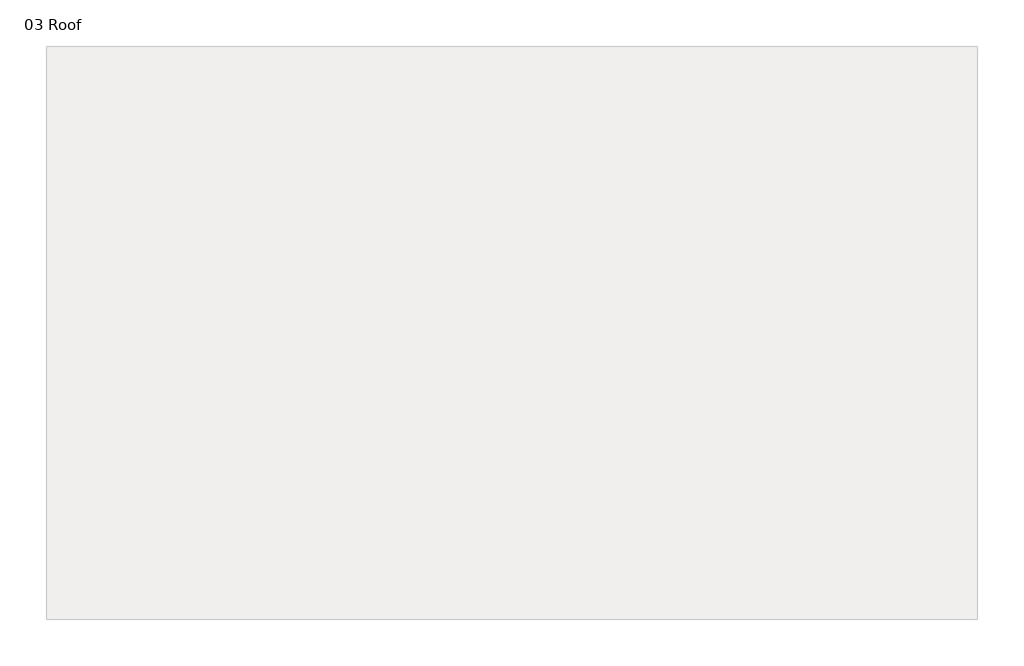
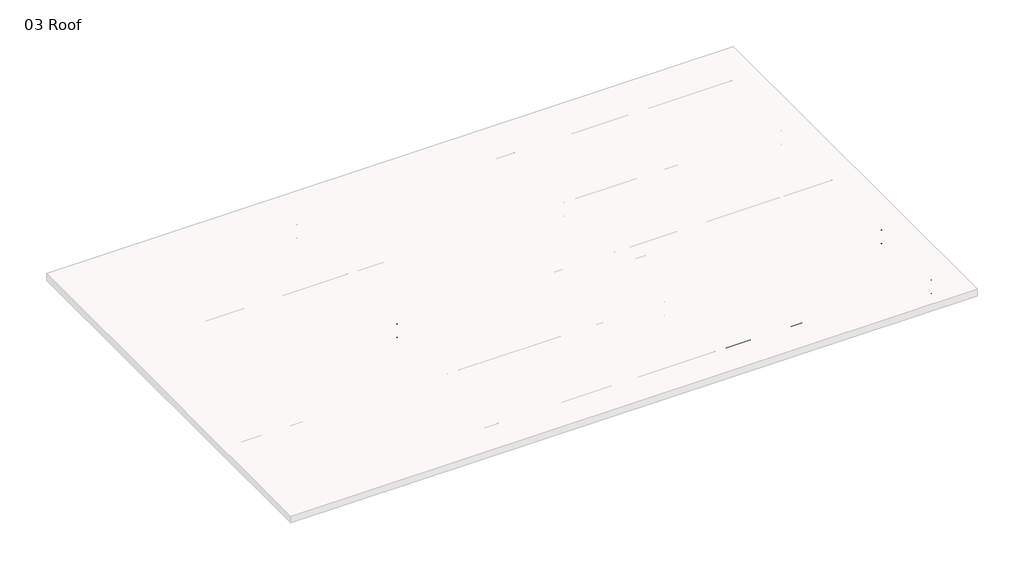
# One storey, part 2 of 4: 101 beams.
"""IFC4 building model written with IfcOpenShell, lengths in millimetres."""

import ifcopenshell
import ifcopenshell.guid

model = None  # the IFC model being written
_history = None  # IfcOwnerHistory: only IFC2X3 demands one
_inside = {}  # id of a spatial element -> (the spatial element, [elements in it])
_under = {}  # id of a project, library or spatial element -> (it, [spatial elements below it])
_declared = {}  # id of a project -> (the project, [libraries it declares])
_typed = {}  # id of a type object -> (the type object, [elements of that type])
_made_of = {}  # id of a material, layer set ... -> (it, [elements and type objects made of it])


def new_model(schema):
    """Start an empty IFC model of exactly this schema.

    Asked for "IFC4X3", IfcOpenShell would pick the latest addendum, in which some entities
    have other attributes; the version numbers below select the first issue.
    IFC2X3 requires an IfcOwnerHistory on every rooted entity: one is made here for all.
    """
    global model, _history
    if schema == "IFC4X3":
        model = ifcopenshell.file(schema_version=(4, 3, 0, 0))
    else:
        model = ifcopenshell.file(schema=schema)
    _inside.clear()
    _under.clear()
    _declared.clear()
    _typed.clear()
    _made_of.clear()
    _history = None
    if model.schema == "IFC2X3":
        org = make("IfcOrganization", Name="unknown")
        user = make(
            "IfcPersonAndOrganization",
            ThePerson=make("IfcPerson", FamilyName="unknown"),
            TheOrganization=org,
        )
        app = make(
            "IfcApplication",
            ApplicationDeveloper=org,
            Version="unknown",
            ApplicationFullName="unknown",
            ApplicationIdentifier="unknown",
        )
        _history = make(
            "IfcOwnerHistory",
            OwningUser=user,
            OwningApplication=app,
            ChangeAction="ADDED",
            CreationDate=0,
        )
    return model


def make(cls, **values):
    """One entity of the class cls with the attributes given. An attribute that is None is left unset."""
    return model.create_entity(
        cls, **{name: value for name, value in values.items() if value is not None}
    )


def rooted(cls, **values):
    """An entity with a GlobalId (a new one), such as an element, a storey or a relation."""
    return make(cls, GlobalId=ifcopenshell.guid.new(), OwnerHistory=_history, **values)


def si_unit(unit_type, name, prefix=None):
    """IfcSIUnit, for example si_unit("LENGTHUNIT", "METRE", prefix="MILLI")."""
    return make("IfcSIUnit", UnitType=unit_type, Prefix=prefix, Name=name)


def assignment(units):
    """IfcUnitAssignment: the units of a project."""
    return None if units is None else make("IfcUnitAssignment", Units=units)


def point(xyz):
    """IfcCartesianPoint."""
    return None if xyz is None else make("IfcCartesianPoint", Coordinates=xyz)


def direction(xyz):
    """IfcDirection."""
    return None if xyz is None else make("IfcDirection", DirectionRatios=xyz)


def frame(location, z_axis=None, x_axis=None):
    """IfcAxis2Placement3D, a coordinate frame: its origin and axes. An axis left out is left unset."""
    return make(
        "IfcAxis2Placement3D",
        Location=point(location),
        Axis=direction(z_axis),
        RefDirection=direction(x_axis),
    )


def frame_2d(location, x_axis=None):
    """IfcAxis2Placement2D, a coordinate frame in the plane: its origin and x axis."""
    return make(
        "IfcAxis2Placement2D", Location=point(location), RefDirection=direction(x_axis)
    )


def origin():
    """The frame at (0, 0, 0) with its axes left unset."""
    return frame((0.0, 0.0, 0.0))


def place(relative_to, where):
    """IfcLocalPlacement: puts the frame where relative to a parent placement (None: the world)."""
    return make(
        "IfcLocalPlacement", PlacementRelTo=relative_to, RelativePlacement=where
    )


def context(
    kind, dimensions, precision=None, world=None, true_north=None, identifier=None
):
    """IfcGeometricRepresentationContext, for example the 3D "Model" context."""
    return make(
        "IfcGeometricRepresentationContext",
        ContextIdentifier=identifier,
        ContextType=kind,
        CoordinateSpaceDimension=dimensions,
        Precision=precision,
        WorldCoordinateSystem=world,
        TrueNorth=true_north,
    )


def project(units=None, contexts=None):
    """IfcProject with its units and contexts."""
    return rooted(
        "IfcProject",
        Name="project",
        RepresentationContexts=contexts,
        UnitsInContext=assignment(units),
    )


def spatial(cls, under=None, at=None, **own):
    """A site, building, storey or space (cls), placed at a placement, below another one or the project."""
    s = rooted(cls, ObjectPlacement=at, **own)
    if under is not None:
        _under.setdefault(under.id(), (under, []))[1].append(s)
    return s


def polyline(points):
    """IfcPolyline through the points."""
    return make("IfcPolyline", Points=[point(p) for p in points])


def circle_curve(where, radius):
    """IfcCircle in the frame where."""
    return make("IfcCircle", Position=where, Radius=radius)


def trimmed(basis, trim1, trim2, sense, master):
    """IfcTrimmedCurve: the piece of a basis curve between two trims."""
    return make(
        "IfcTrimmedCurve",
        BasisCurve=basis,
        Trim1=trim1,
        Trim2=trim2,
        SenseAgreement=sense,
        MasterRepresentation=master,
    )


def segment(curve, same_sense, transition):
    """IfcCompositeCurveSegment."""
    return make(
        "IfcCompositeCurveSegment",
        Transition=transition,
        SameSense=same_sense,
        ParentCurve=curve,
    )


def composite_curve(segments, self_intersect=None):
    """IfcCompositeCurve: segments joined end to end."""
    return make("IfcCompositeCurve", Segments=segments, SelfIntersect=self_intersect)


def outline(outer, holes=None, kind="AREA"):
    """IfcArbitraryClosedProfileDef: a profile drawn as a closed curve; with holes, ...WithVoids."""
    if holes is None:
        return make("IfcArbitraryClosedProfileDef", ProfileType=kind, OuterCurve=outer)
    return make(
        "IfcArbitraryProfileDefWithVoids",
        ProfileType=kind,
        OuterCurve=outer,
        InnerCurves=holes,
    )


def extrude(swept, where, along, depth):
    """IfcExtrudedAreaSolid: the profile swept, set in the frame where, extruded along a direction by depth."""
    return make(
        "IfcExtrudedAreaSolid",
        SweptArea=swept,
        Position=where,
        ExtrudedDirection=direction(along),
        Depth=depth,
    )


def shape(context_of_items, identifier, shape_type, items):
    """IfcShapeRepresentation: the items that make up one representation, for example the "Body"."""
    return make(
        "IfcShapeRepresentation",
        ContextOfItems=context_of_items,
        RepresentationIdentifier=identifier,
        RepresentationType=shape_type,
        Items=items,
    )


def source(mapping_origin, context_of_items, identifier, shape_type, items):
    """IfcRepresentationMap: a shape defined once, which mapped items show again and again."""
    return make(
        "IfcRepresentationMap",
        MappingOrigin=mapping_origin,
        MappedRepresentation=shape(context_of_items, identifier, shape_type, items),
    )


def transform(
    local_origin,
    x_axis=None,
    y_axis=None,
    z_axis=None,
    scale=None,
    scale2=None,
    scale3=None,
    uniform=True,
):
    """IfcCartesianTransformationOperator3D, or its non-uniform kind. x_axis, y_axis, z_axis: its Axis1, 2, 3."""
    if uniform:
        return make(
            "IfcCartesianTransformationOperator3D",
            Axis1=direction(x_axis),
            Axis2=direction(y_axis),
            LocalOrigin=point(local_origin),
            Scale=scale,
            Axis3=direction(z_axis),
        )
    return make(
        "IfcCartesianTransformationOperator3DnonUniform",
        Axis1=direction(x_axis),
        Axis2=direction(y_axis),
        LocalOrigin=point(local_origin),
        Scale=scale,
        Axis3=direction(z_axis),
        Scale2=scale2,
        Scale3=scale3,
    )


def mapped(mapping_source, mapping_target):
    """IfcMappedItem: shows the shape of a source again, moved by a transform."""
    return make(
        "IfcMappedItem", MappingSource=mapping_source, MappingTarget=mapping_target
    )


def made_of(thing, what):
    """Note that an element or type object is made of a material, layer set ...; save() writes the relation."""
    if what is not None:
        _made_of.setdefault(what.id(), (what, []))[1].append(thing)
    return thing


def element(
    cls,
    number,
    at=None,
    inside=None,
    cuts=None,
    type_object=None,
    material=None,
    context=None,
    identifier="Body",
    shape_type=None,
    held_by="IfcProductDefinitionShape",
    body=None,
    shapes=None,
    **own,
):
    """One element of the class cls, such as IfcWall. Its Tag is "e" and its number.

    at: its placement. inside: the storey or other place that contains it. cuts: it is an
    opening in that element (IfcRelVoidsElement). A single representation is given by context,
    identifier, shape_type and body (its items); several are given by shapes. held_by: the class
    of the entity that holds the representations. save() writes the other relations.
    """
    e = rooted(cls, Tag="e%d" % number, ObjectPlacement=at, **own)
    if body is not None:
        shapes = [shape(context, identifier, shape_type, body)]
    if shapes is not None:
        e.Representation = make(held_by, Representations=shapes)
    if inside is not None:
        _inside.setdefault(inside.id(), (inside, []))[1].append(e)
    if cuts is not None:
        rooted(
            "IfcRelVoidsElement", RelatingBuildingElement=cuts, RelatedOpeningElement=e
        )
    if type_object is not None:
        _typed.setdefault(type_object.id(), (type_object, []))[1].append(e)
    return made_of(e, material)


def aggregate(whole, parts):
    """IfcRelAggregates: a whole, such as a stair, and the parts it consists of."""
    return rooted("IfcRelAggregates", RelatingObject=whole, RelatedObjects=parts)


def save(model, path):
    """Write the relations noted so far, then the file.

    IfcRelAggregates (storeys below a building ...), IfcRelContainedInSpatialStructure (elements
    in a storey), IfcRelDefinesByType, IfcRelAssociatesMaterial and IfcRelDeclares: one each for
    every whole, place, type object, material and project.
    """
    for whole, parts in _under.values():
        aggregate(whole, parts)
    for where, things in _inside.values():
        rooted(
            "IfcRelContainedInSpatialStructure",
            RelatedElements=things,
            RelatingStructure=where,
        )
    for kind, things in _typed.values():
        rooted("IfcRelDefinesByType", RelatedObjects=things, RelatingType=kind)
    for what, things in _made_of.values():
        rooted("IfcRelAssociatesMaterial", RelatedObjects=things, RelatingMaterial=what)
    for by, libraries in _declared.values():
        rooted("IfcRelDeclares", RelatingContext=by, RelatedDefinitions=libraries)
    model.write(path)


def ub_universal_beam_305x165x40ub_24de31be(model_context):
    return source(origin(), model_context, "Body", "SweptSolid", [
        extrude(outline(composite_curve([segment(polyline([(82.5, -141.5), (82.5, -151.7), (-82.5, -151.7), (-82.5, -141.5), (-11.9, -141.5)]), True, "CONTINUOUS"), segment(trimmed(circle_curve(frame_2d((-11.9, -132.6)), 8.9), [point((-11.9, -141.5))], [point((-3.0, -132.6))], True, "CARTESIAN"), True, "CONTINUOUS"), segment(polyline([(-3.0, -132.6), (-3.0, 132.6)]), True, "CONTINUOUS"), segment(trimmed(circle_curve(frame_2d((-11.9, 132.6)), 8.9), [point((-3.0, 132.6))], [point((-11.9, 141.5))], True, "CARTESIAN"), True, "CONTINUOUS"), segment(polyline([(-11.9, 141.5), (-82.5, 141.5), (-82.5, 151.7), (82.5, 151.7), (82.5, 141.5), (11.9, 141.5)]), True, "CONTINUOUS"), segment(trimmed(circle_curve(frame_2d((11.9, 132.6)), 8.9), [point((11.9, 141.5))], [point((3.0, 132.6))], True, "CARTESIAN"), True, "CONTINUOUS"), segment(polyline([(3.0, 132.6), (3.0, -132.6)]), True, "CONTINUOUS"), segment(trimmed(circle_curve(frame_2d((11.9, -132.6)), 8.9), [point((3.0, -132.6))], [point((11.9, -141.5))], True, "CARTESIAN"), True, "CONTINUOUS"), segment(polyline([(11.9, -141.5), (82.5, -141.5)]), True, "CONTINUOUS")], self_intersect=False)), frame((-335.6, 0.0, 0.0), z_axis=(1.0, 0.0, 0.0), x_axis=(0.0, 1.0, 0.0)), (0.0, 0.0, 1.0), 671.2),
    ])


def ub_universal_beam_305x165x40ub_f67fc52f(model_context):
    return source(origin(), model_context, "Body", "SweptSolid", [
        extrude(outline(composite_curve([segment(polyline([(82.5, -141.5), (82.5, -151.7), (-82.5, -151.7), (-82.5, -141.5), (-11.9, -141.5)]), True, "CONTINUOUS"), segment(trimmed(circle_curve(frame_2d((-11.9, -132.6)), 8.9), [point((-11.9, -141.5))], [point((-3.0, -132.6))], True, "CARTESIAN"), True, "CONTINUOUS"), segment(polyline([(-3.0, -132.6), (-3.0, 132.6)]), True, "CONTINUOUS"), segment(trimmed(circle_curve(frame_2d((-11.9, 132.6)), 8.9), [point((-3.0, 132.6))], [point((-11.9, 141.5))], True, "CARTESIAN"), True, "CONTINUOUS"), segment(polyline([(-11.9, 141.5), (-82.5, 141.5), (-82.5, 151.7), (82.5, 151.7), (82.5, 141.5), (11.9, 141.5)]), True, "CONTINUOUS"), segment(trimmed(circle_curve(frame_2d((11.9, 132.6)), 8.9), [point((11.9, 141.5))], [point((3.0, 132.6))], True, "CARTESIAN"), True, "CONTINUOUS"), segment(polyline([(3.0, 132.6), (3.0, -132.6)]), True, "CONTINUOUS"), segment(trimmed(circle_curve(frame_2d((11.9, -132.6)), 8.9), [point((3.0, -132.6))], [point((11.9, -141.5))], True, "CARTESIAN"), True, "CONTINUOUS"), segment(polyline([(11.9, -141.5), (82.5, -141.5)]), True, "CONTINUOUS")], self_intersect=False)), frame((-7125.0, 0.0, 0.0), z_axis=(1.0, 0.0, 0.0), x_axis=(0.0, 1.0, 0.0)), (0.0, 0.0, 1.0), 14250.0),
    ])


def ub_universal_beam_305x165x40ub_26fb8d3a(model_context):
    return source(origin(), model_context, "Body", "SweptSolid", [
        extrude(outline(composite_curve([segment(polyline([(82.5, -141.5), (82.5, -151.7), (-82.5, -151.7), (-82.5, -141.5), (-11.9, -141.5)]), True, "CONTINUOUS"), segment(trimmed(circle_curve(frame_2d((-11.9, -132.6)), 8.9), [point((-11.9, -141.5))], [point((-3.0, -132.6))], True, "CARTESIAN"), True, "CONTINUOUS"), segment(polyline([(-3.0, -132.6), (-3.0, 132.6)]), True, "CONTINUOUS"), segment(trimmed(circle_curve(frame_2d((-11.9, 132.6)), 8.9), [point((-3.0, 132.6))], [point((-11.9, 141.5))], True, "CARTESIAN"), True, "CONTINUOUS"), segment(polyline([(-11.9, 141.5), (-82.5, 141.5), (-82.5, 151.7), (82.5, 151.7), (82.5, 141.5), (11.9, 141.5)]), True, "CONTINUOUS"), segment(trimmed(circle_curve(frame_2d((11.9, 132.6)), 8.9), [point((11.9, 141.5))], [point((3.0, 132.6))], True, "CARTESIAN"), True, "CONTINUOUS"), segment(polyline([(3.0, 132.6), (3.0, -132.6)]), True, "CONTINUOUS"), segment(trimmed(circle_curve(frame_2d((11.9, -132.6)), 8.9), [point((3.0, -132.6))], [point((11.9, -141.5))], True, "CARTESIAN"), True, "CONTINUOUS"), segment(polyline([(11.9, -141.5), (82.5, -141.5)]), True, "CONTINUOUS")], self_intersect=False)), frame((-347.8807825, 0.0, 0.0), z_axis=(1.0, 0.0, 0.0), x_axis=(0.0, 1.0, 0.0)), (0.0, 0.0, 1.0), 695.761565),
    ])


model = new_model("IFC4")

# Units and contexts
model_context = context("Model", 3, world=origin())
ifc_project = project(units=[si_unit("LENGTHUNIT", "METRE", prefix="MILLI")], contexts=[model_context])

# Site, building, storey
site = spatial("IfcSite", under=ifc_project)
building = spatial("IfcBuilding", under=site)
storey = spatial("IfcBuildingStorey", under=building, Name="03 Roof", Elevation=8000.0)

# Beams
placement = place(None, origin())
ub_universal_beam_305x165x40ub_shape = ub_universal_beam_305x165x40ub_24de31be(model_context)
element("IfcBeam", 1, ObjectType="UB-Universal Beam : 305x165x40UB", at=placement, inside=storey, context=model_context, shape_type="MappedRepresentation", body=[
    mapped(ub_universal_beam_305x165x40ub_shape, transform((-21151.5506826, 12261.9474871, 7500.0), x_axis=(0.0, 0.0, 1.0), y_axis=(0.0, -1.0, 0.0), z_axis=(1.0, 0.0, 0.0))),
])
element("IfcBeam", 2, ObjectType="UB-Universal Beam : 305x165x40UB", at=placement, inside=storey, context=model_context, shape_type="MappedRepresentation", body=[
    mapped(ub_universal_beam_305x165x40ub_shape, transform((-19964.0506826, 12261.9474871, 7500.0), x_axis=(0.0, 0.0, 1.0), y_axis=(0.0, -1.0, 0.0), z_axis=(1.0, 0.0, 0.0))),
])
element("IfcBeam", 3, ObjectType="UB-Universal Beam : 305x165x40UB", at=placement, inside=storey, context=model_context, shape_type="MappedRepresentation", body=[
    mapped(ub_universal_beam_305x165x40ub_shape, transform((-18776.5506826, 12261.9474871, 7500.0), x_axis=(0.0, 0.0, 1.0), y_axis=(0.0, -1.0, 0.0), z_axis=(1.0, 0.0, 0.0))),
])
element("IfcBeam", 4, ObjectType="UB-Universal Beam : 305x165x40UB", at=placement, inside=storey, context=model_context, shape_type="MappedRepresentation", body=[
    mapped(ub_universal_beam_305x165x40ub_shape, transform((-17589.0506826, 12261.9474871, 7500.0), x_axis=(0.0, 0.0, 1.0), y_axis=(0.0, -1.0, 0.0), z_axis=(1.0, 0.0, 0.0))),
])
element("IfcBeam", 5, ObjectType="UB-Universal Beam : 305x165x40UB", at=placement, inside=storey, context=model_context, shape_type="MappedRepresentation", body=[
    mapped(ub_universal_beam_305x165x40ub_shape, transform((-22339.0506826, 12261.9474871, 7500.0), x_axis=(0.0, 0.0, 1.0), y_axis=(0.0, -1.0, 0.0), z_axis=(1.0, 0.0, 0.0))),
])
element("IfcBeam", 6, ObjectType="UB-Universal Beam : 305x165x40UB", at=placement, inside=storey, context=model_context, shape_type="MappedRepresentation", body=[
    mapped(ub_universal_beam_305x165x40ub_shape, transform((-16401.5506826, 12261.9474871, 7500.0), x_axis=(0.0, 0.0, 1.0), y_axis=(0.0, -1.0, 0.0), z_axis=(1.0, 0.0, 0.0))),
])
element("IfcBeam", 7, ObjectType="UB-Universal Beam : 305x165x40UB", at=placement, inside=storey, context=model_context, shape_type="MappedRepresentation", body=[
    mapped(ub_universal_beam_305x165x40ub_shape, transform((-21151.5506826, 6271.8474871, 7500.0), x_axis=(0.0, 0.0, 1.0), y_axis=(0.0, -1.0, 0.0), z_axis=(1.0, 0.0, 0.0))),
])
element("IfcBeam", 8, ObjectType="UB-Universal Beam : 305x165x40UB", at=placement, inside=storey, context=model_context, shape_type="MappedRepresentation", body=[
    mapped(ub_universal_beam_305x165x40ub_shape, transform((-19964.0506826, 6271.8474871, 7500.0), x_axis=(0.0, 0.0, 1.0), y_axis=(0.0, -1.0, 0.0), z_axis=(1.0, 0.0, 0.0))),
])
element("IfcBeam", 9, ObjectType="UB-Universal Beam : 305x165x40UB", at=placement, inside=storey, context=model_context, shape_type="MappedRepresentation", body=[
    mapped(ub_universal_beam_305x165x40ub_shape, transform((-18776.5506826, 6271.8474871, 7500.0), x_axis=(0.0, 0.0, 1.0), y_axis=(0.0, -1.0, 0.0), z_axis=(1.0, 0.0, 0.0))),
])
element("IfcBeam", 10, ObjectType="UB-Universal Beam : 305x165x40UB", at=placement, inside=storey, context=model_context, shape_type="MappedRepresentation", body=[
    mapped(ub_universal_beam_305x165x40ub_shape, transform((-17589.0506826, 6271.8474871, 7500.0), x_axis=(0.0, 0.0, 1.0), y_axis=(0.0, -1.0, 0.0), z_axis=(1.0, 0.0, 0.0))),
])
element("IfcBeam", 11, ObjectType="UB-Universal Beam : 305x165x40UB", at=placement, inside=storey, context=model_context, shape_type="MappedRepresentation", body=[
    mapped(ub_universal_beam_305x165x40ub_shape, transform((-22339.0506826, 6271.8474871, 7500.0), x_axis=(0.0, 0.0, 1.0), y_axis=(0.0, -1.0, 0.0), z_axis=(1.0, 0.0, 0.0))),
])
element("IfcBeam", 12, ObjectType="UB-Universal Beam : 305x165x40UB", at=placement, inside=storey, context=model_context, shape_type="MappedRepresentation", body=[
    mapped(ub_universal_beam_305x165x40ub_shape, transform((-16401.5506826, 6271.8474871, 7500.0), x_axis=(0.0, 0.0, 1.0), y_axis=(0.0, -1.0, 0.0), z_axis=(1.0, 0.0, 0.0))),
])
element("IfcBeam", 13, ObjectType="UB-Universal Beam : 305x165x40UB", at=placement, inside=storey, context=model_context, shape_type="MappedRepresentation", body=[
    mapped(ub_universal_beam_305x165x40ub_shape, transform((20723.4493174, -5728.1525129, 7500.0), x_axis=(0.0, 0.0, 1.0), y_axis=(0.0, -1.0, 0.0), z_axis=(1.0, 0.0, 0.0))),
])
element("IfcBeam", 14, ObjectType="UB-Universal Beam : 305x165x40UB", at=placement, inside=storey, context=model_context, shape_type="MappedRepresentation", body=[
    mapped(ub_universal_beam_305x165x40ub_shape, transform((8848.4493174, -5728.1525129, 7500.0), x_axis=(0.0, 0.0, 1.0), y_axis=(0.0, -1.0, 0.0), z_axis=(1.0, 0.0, 0.0))),
])
element("IfcBeam", 15, ObjectType="UB-Universal Beam : 305x165x40UB", at=placement, inside=storey, context=model_context, shape_type="MappedRepresentation", body=[
    mapped(ub_universal_beam_305x165x40ub_shape, transform((19535.9493174, -5728.1525129, 7500.0), x_axis=(0.0, 0.0, 1.0), y_axis=(0.0, -1.0, 0.0), z_axis=(1.0, 0.0, 0.0))),
])
element("IfcBeam", 16, ObjectType="UB-Universal Beam : 305x165x40UB", at=placement, inside=storey, context=model_context, shape_type="MappedRepresentation", body=[
    mapped(ub_universal_beam_305x165x40ub_shape, transform((10035.9493174, -5728.1525129, 7500.0), x_axis=(0.0, 0.0, 1.0), y_axis=(0.0, -1.0, 0.0), z_axis=(1.0, 0.0, 0.0))),
])
element("IfcBeam", 17, ObjectType="UB-Universal Beam : 305x165x40UB", at=placement, inside=storey, context=model_context, shape_type="MappedRepresentation", body=[
    mapped(ub_universal_beam_305x165x40ub_shape, transform((18348.4493174, -5728.1525129, 7500.0), x_axis=(0.0, 0.0, 1.0), y_axis=(0.0, -1.0, 0.0), z_axis=(1.0, 0.0, 0.0))),
])
element("IfcBeam", 18, ObjectType="UB-Universal Beam : 305x165x40UB", at=placement, inside=storey, context=model_context, shape_type="MappedRepresentation", body=[
    mapped(ub_universal_beam_305x165x40ub_shape, transform((17160.9493174, -5728.1525129, 7500.0), x_axis=(0.0, 0.0, 1.0), y_axis=(0.0, -1.0, 0.0), z_axis=(1.0, 0.0, 0.0))),
])
element("IfcBeam", 19, ObjectType="UB-Universal Beam : 305x165x40UB", at=placement, inside=storey, context=model_context, shape_type="MappedRepresentation", body=[
    mapped(ub_universal_beam_305x165x40ub_shape, transform((21910.9493174, -5728.1525129, 7500.0), x_axis=(0.0, 0.0, 1.0), y_axis=(0.0, -1.0, 0.0), z_axis=(1.0, 0.0, 0.0))),
])
element("IfcBeam", 20, ObjectType="UB-Universal Beam : 305x165x40UB", at=placement, inside=storey, context=model_context, shape_type="MappedRepresentation", body=[
    mapped(ub_universal_beam_305x165x40ub_shape, transform((15973.4493174, -5728.1525129, 7500.0), x_axis=(0.0, 0.0, 1.0), y_axis=(0.0, -1.0, 0.0), z_axis=(1.0, 0.0, 0.0))),
])
element("IfcBeam", 21, ObjectType="UB-Universal Beam : 305x165x40UB", at=placement, inside=storey, context=model_context, shape_type="MappedRepresentation", body=[
    mapped(ub_universal_beam_305x165x40ub_shape, transform((11223.4493174, -5728.1525129, 7500.0), x_axis=(0.0, 0.0, 1.0), y_axis=(0.0, -1.0, 0.0), z_axis=(1.0, 0.0, 0.0))),
])
element("IfcBeam", 22, ObjectType="UB-Universal Beam : 305x165x40UB", at=placement, inside=storey, context=model_context, shape_type="MappedRepresentation", body=[
    mapped(ub_universal_beam_305x165x40ub_shape, transform((12410.9493174, -5728.1525129, 7500.0), x_axis=(0.0, 0.0, 1.0), y_axis=(0.0, -1.0, 0.0), z_axis=(1.0, 0.0, 0.0))),
])
element("IfcBeam", 23, ObjectType="UB-Universal Beam : 305x165x40UB", at=placement, inside=storey, context=model_context, shape_type="MappedRepresentation", body=[
    mapped(ub_universal_beam_305x165x40ub_shape, transform((7660.9493174, -5728.1525129, 7500.0), x_axis=(0.0, 0.0, 1.0), y_axis=(0.0, -1.0, 0.0), z_axis=(1.0, 0.0, 0.0))),
])
element("IfcBeam", 24, ObjectType="UB-Universal Beam : 305x165x40UB", at=placement, inside=storey, context=model_context, shape_type="MappedRepresentation", body=[
    mapped(ub_universal_beam_305x165x40ub_shape, transform((13598.4493174, -5728.1525129, 7500.0), x_axis=(0.0, 0.0, 1.0), y_axis=(0.0, -1.0, 0.0), z_axis=(1.0, 0.0, 0.0))),
])
element("IfcBeam", 25, ObjectType="UB-Universal Beam : 305x165x40UB", at=placement, inside=storey, context=model_context, shape_type="MappedRepresentation", body=[
    mapped(ub_universal_beam_305x165x40ub_shape, transform((14785.9493174, -5728.1525129, 7500.0), x_axis=(0.0, 0.0, 1.0), y_axis=(0.0, -1.0, 0.0), z_axis=(1.0, 0.0, 0.0))),
])
element("IfcBeam", 26, ObjectType="UB-Universal Beam : 305x165x40UB", at=placement, inside=storey, context=model_context, shape_type="MappedRepresentation", body=[
    mapped(ub_universal_beam_305x165x40ub_shape, transform((20723.4493174, -11728.1525129, 7500.0), x_axis=(0.0, 0.0, 1.0), y_axis=(0.0, -1.0, 0.0), z_axis=(1.0, 0.0, 0.0))),
])
element("IfcBeam", 27, ObjectType="UB-Universal Beam : 305x165x40UB", at=placement, inside=storey, context=model_context, shape_type="MappedRepresentation", body=[
    mapped(ub_universal_beam_305x165x40ub_shape, transform((19535.9493174, -11728.1525129, 7500.0), x_axis=(0.0, 0.0, 1.0), y_axis=(0.0, -1.0, 0.0), z_axis=(1.0, 0.0, 0.0))),
])
element("IfcBeam", 28, ObjectType="UB-Universal Beam : 305x165x40UB", at=placement, inside=storey, context=model_context, shape_type="MappedRepresentation", body=[
    mapped(ub_universal_beam_305x165x40ub_shape, transform((10035.9493174, -11728.1525129, 7500.0), x_axis=(0.0, 0.0, 1.0), y_axis=(0.0, -1.0, 0.0), z_axis=(1.0, 0.0, 0.0))),
])
element("IfcBeam", 29, ObjectType="UB-Universal Beam : 305x165x40UB", at=placement, inside=storey, context=model_context, shape_type="MappedRepresentation", body=[
    mapped(ub_universal_beam_305x165x40ub_shape, transform((18348.4493174, -11728.1525129, 7500.0), x_axis=(0.0, 0.0, 1.0), y_axis=(0.0, -1.0, 0.0), z_axis=(1.0, 0.0, 0.0))),
])
element("IfcBeam", 30, ObjectType="UB-Universal Beam : 305x165x40UB", at=placement, inside=storey, context=model_context, shape_type="MappedRepresentation", body=[
    mapped(ub_universal_beam_305x165x40ub_shape, transform((17160.9493174, -11728.1525129, 7500.0), x_axis=(0.0, 0.0, 1.0), y_axis=(0.0, -1.0, 0.0), z_axis=(1.0, 0.0, 0.0))),
])
element("IfcBeam", 31, ObjectType="UB-Universal Beam : 305x165x40UB", at=placement, inside=storey, context=model_context, shape_type="MappedRepresentation", body=[
    mapped(ub_universal_beam_305x165x40ub_shape, transform((21910.9493174, -11728.1525129, 7500.0), x_axis=(0.0, 0.0, 1.0), y_axis=(0.0, -1.0, 0.0), z_axis=(1.0, 0.0, 0.0))),
])
element("IfcBeam", 32, ObjectType="UB-Universal Beam : 305x165x40UB", at=placement, inside=storey, context=model_context, shape_type="MappedRepresentation", body=[
    mapped(ub_universal_beam_305x165x40ub_shape, transform((15973.4493174, -11728.1525129, 7500.0), x_axis=(0.0, 0.0, 1.0), y_axis=(0.0, -1.0, 0.0), z_axis=(1.0, 0.0, 0.0))),
])
element("IfcBeam", 33, ObjectType="UB-Universal Beam : 305x165x40UB", at=placement, inside=storey, context=model_context, shape_type="MappedRepresentation", body=[
    mapped(ub_universal_beam_305x165x40ub_shape, transform((11223.4493174, -11728.1525129, 7500.0), x_axis=(0.0, 0.0, 1.0), y_axis=(0.0, -1.0, 0.0), z_axis=(1.0, 0.0, 0.0))),
])
element("IfcBeam", 34, ObjectType="UB-Universal Beam : 305x165x40UB", at=placement, inside=storey, context=model_context, shape_type="MappedRepresentation", body=[
    mapped(ub_universal_beam_305x165x40ub_shape, transform((12410.9493174, -11728.1525129, 7500.0), x_axis=(0.0, 0.0, 1.0), y_axis=(0.0, -1.0, 0.0), z_axis=(1.0, 0.0, 0.0))),
])
element("IfcBeam", 35, ObjectType="UB-Universal Beam : 305x165x40UB", at=placement, inside=storey, context=model_context, shape_type="MappedRepresentation", body=[
    mapped(ub_universal_beam_305x165x40ub_shape, transform((13598.4493174, -11728.1525129, 7500.0), x_axis=(0.0, 0.0, 1.0), y_axis=(0.0, -1.0, 0.0), z_axis=(1.0, 0.0, 0.0))),
])
element("IfcBeam", 36, ObjectType="UB-Universal Beam : 305x165x40UB", at=placement, inside=storey, context=model_context, shape_type="MappedRepresentation", body=[
    mapped(ub_universal_beam_305x165x40ub_shape, transform((14785.9493174, -11728.1525129, 7500.0), x_axis=(0.0, 0.0, 1.0), y_axis=(0.0, -1.0, 0.0), z_axis=(1.0, 0.0, 0.0))),
])
element("IfcBeam", 37, ObjectType="UB-Universal Beam : 305x165x40UB", at=placement, inside=storey, context=model_context, shape_type="MappedRepresentation", body=[
    mapped(ub_universal_beam_305x165x40ub_shape, transform((5723.4493174, -5728.1525129, 7500.0), x_axis=(0.0, 0.0, 1.0), y_axis=(0.0, -1.0, 0.0), z_axis=(1.0, 0.0, 0.0))),
])
element("IfcBeam", 38, ObjectType="UB-Universal Beam : 305x165x40UB", at=placement, inside=storey, context=model_context, shape_type="MappedRepresentation", body=[
    mapped(ub_universal_beam_305x165x40ub_shape, transform((4535.9493174, -5728.1525129, 7500.0), x_axis=(0.0, 0.0, 1.0), y_axis=(0.0, -1.0, 0.0), z_axis=(1.0, 0.0, 0.0))),
])
element("IfcBeam", 39, ObjectType="UB-Universal Beam : 305x165x40UB", at=placement, inside=storey, context=model_context, shape_type="MappedRepresentation", body=[
    mapped(ub_universal_beam_305x165x40ub_shape, transform((3348.4493174, -5728.1525129, 7500.0), x_axis=(0.0, 0.0, 1.0), y_axis=(0.0, -1.0, 0.0), z_axis=(1.0, 0.0, 0.0))),
])
element("IfcBeam", 40, ObjectType="UB-Universal Beam : 305x165x40UB", at=placement, inside=storey, context=model_context, shape_type="MappedRepresentation", body=[
    mapped(ub_universal_beam_305x165x40ub_shape, transform((2160.9493174, -5728.1525129, 7500.0), x_axis=(0.0, 0.0, 1.0), y_axis=(0.0, -1.0, 0.0), z_axis=(1.0, 0.0, 0.0))),
])
element("IfcBeam", 41, ObjectType="UB-Universal Beam : 305x165x40UB", at=placement, inside=storey, context=model_context, shape_type="MappedRepresentation", body=[
    mapped(ub_universal_beam_305x165x40ub_shape, transform((6910.9493174, -5728.1525129, 7500.0), x_axis=(0.0, 0.0, 1.0), y_axis=(0.0, -1.0, 0.0), z_axis=(1.0, 0.0, 0.0))),
])
element("IfcBeam", 42, ObjectType="UB-Universal Beam : 305x165x40UB", at=placement, inside=storey, context=model_context, shape_type="MappedRepresentation", body=[
    mapped(ub_universal_beam_305x165x40ub_shape, transform((973.4493174, -5728.1525129, 7500.0), x_axis=(0.0, 0.0, 1.0), y_axis=(0.0, -1.0, 0.0), z_axis=(1.0, 0.0, 0.0))),
])
element("IfcBeam", 43, ObjectType="UB-Universal Beam : 305x165x40UB", at=placement, inside=storey, context=model_context, shape_type="MappedRepresentation", body=[
    mapped(ub_universal_beam_305x165x40ub_shape, transform((-21151.5506826, 271.8474871, 7500.0), x_axis=(0.0, 0.0, 1.0), y_axis=(0.0, -1.0, 0.0), z_axis=(1.0, 0.0, 0.0))),
])
element("IfcBeam", 44, ObjectType="UB-Universal Beam : 305x165x40UB", at=placement, inside=storey, context=model_context, shape_type="MappedRepresentation", body=[
    mapped(ub_universal_beam_305x165x40ub_shape, transform((-19964.0506826, 271.8474871, 7500.0), x_axis=(0.0, 0.0, 1.0), y_axis=(0.0, -1.0, 0.0), z_axis=(1.0, 0.0, 0.0))),
])
element("IfcBeam", 45, ObjectType="UB-Universal Beam : 305x165x40UB", at=placement, inside=storey, context=model_context, shape_type="MappedRepresentation", body=[
    mapped(ub_universal_beam_305x165x40ub_shape, transform((-14026.5506826, 271.8474871, 7500.0), x_axis=(0.0, 0.0, 1.0), y_axis=(0.0, -1.0, 0.0), z_axis=(1.0, 0.0, 0.0))),
])
element("IfcBeam", 46, ObjectType="UB-Universal Beam : 305x165x40UB", at=placement, inside=storey, context=model_context, shape_type="MappedRepresentation", body=[
    mapped(ub_universal_beam_305x165x40ub_shape, transform((-18776.5506826, 271.8474871, 7500.0), x_axis=(0.0, 0.0, 1.0), y_axis=(0.0, -1.0, 0.0), z_axis=(1.0, 0.0, 0.0))),
])
element("IfcBeam", 47, ObjectType="UB-Universal Beam : 305x165x40UB", at=placement, inside=storey, context=model_context, shape_type="MappedRepresentation", body=[
    mapped(ub_universal_beam_305x165x40ub_shape, transform((-17589.0506826, 271.8474871, 7500.0), x_axis=(0.0, 0.0, 1.0), y_axis=(0.0, -1.0, 0.0), z_axis=(1.0, 0.0, 0.0))),
])
element("IfcBeam", 48, ObjectType="UB-Universal Beam : 305x165x40UB", at=placement, inside=storey, context=model_context, shape_type="MappedRepresentation", body=[
    mapped(ub_universal_beam_305x165x40ub_shape, transform((-22339.0506826, 271.8474871, 7500.0), x_axis=(0.0, 0.0, 1.0), y_axis=(0.0, -1.0, 0.0), z_axis=(1.0, 0.0, 0.0))),
])
element("IfcBeam", 49, ObjectType="UB-Universal Beam : 305x165x40UB", at=placement, inside=storey, context=model_context, shape_type="MappedRepresentation", body=[
    mapped(ub_universal_beam_305x165x40ub_shape, transform((-16401.5506826, 271.8474871, 7500.0), x_axis=(0.0, 0.0, 1.0), y_axis=(0.0, -1.0, 0.0), z_axis=(1.0, 0.0, 0.0))),
])
element("IfcBeam", 50, ObjectType="UB-Universal Beam : 305x165x40UB", at=placement, inside=storey, context=model_context, shape_type="MappedRepresentation", body=[
    mapped(ub_universal_beam_305x165x40ub_shape, transform((-15214.0506826, 271.8474871, 7500.0), x_axis=(0.0, 0.0, 1.0), y_axis=(0.0, -1.0, 0.0), z_axis=(1.0, 0.0, 0.0))),
])
ub_universal_beam_305x165x40ub_2_shape = ub_universal_beam_305x165x40ub_f67fc52f(model_context)
element("IfcBeam", 51, ObjectType="UB-Universal Beam : 305x165x40UB", at=placement, inside=storey, context=model_context, shape_type="MappedRepresentation", body=[
    mapped(ub_universal_beam_305x165x40ub_2_shape, transform((14785.9493174, -5728.1525129, 7000.0), x_axis=(1.0, 0.0, 0.0), y_axis=(0.0, 1.0, 0.0), z_axis=(0.0, 0.0, 1.0))),
])
element("IfcBeam", 52, ObjectType="UB-Universal Beam : 305x165x40UB", at=placement, inside=storey, context=model_context, shape_type="MappedRepresentation", body=[
    mapped(ub_universal_beam_305x165x40ub_2_shape, transform((14785.9493174, -5728.1525129, 8000.0), x_axis=(1.0, 0.0, 0.0), y_axis=(0.0, 1.0, 0.0), z_axis=(0.0, 0.0, 1.0))),
])
element("IfcBeam", 53, ObjectType="UB-Universal Beam : 305x165x40UB", at=placement, inside=storey, context=model_context, shape_type="MappedRepresentation", body=[
    mapped(ub_universal_beam_305x165x40ub_2_shape, transform((14785.9493174, -11728.1525129, 7000.0), x_axis=(1.0, 0.0, 0.0), y_axis=(0.0, 1.0, 0.0), z_axis=(0.0, 0.0, 1.0))),
])
element("IfcBeam", 54, ObjectType="UB-Universal Beam : 305x165x40UB", at=placement, inside=storey, context=model_context, shape_type="MappedRepresentation", body=[
    mapped(ub_universal_beam_305x165x40ub_2_shape, transform((14785.9493174, -11728.1525129, 8000.0), x_axis=(1.0, 0.0, 0.0), y_axis=(0.0, 1.0, 0.0), z_axis=(0.0, 0.0, 1.0))),
])
element("IfcBeam", 55, ObjectType="UB-Universal Beam : 305x165x40UB", at=placement, inside=storey, context=model_context, shape_type="MappedRepresentation", body=[
    mapped(ub_universal_beam_305x165x40ub_2_shape, transform((-15214.0506826, 271.8474871, 7000.0), x_axis=(1.0, 0.0, 0.0), y_axis=(0.0, 1.0, 0.0), z_axis=(0.0, 0.0, 1.0))),
])
element("IfcBeam", 56, ObjectType="UB-Universal Beam : 305x165x40UB", at=placement, inside=storey, context=model_context, shape_type="MappedRepresentation", body=[
    mapped(ub_universal_beam_305x165x40ub_2_shape, transform((-15214.0506826, 271.8474871, 8000.0), x_axis=(1.0, 0.0, 0.0), y_axis=(0.0, 1.0, 0.0), z_axis=(0.0, 0.0, 1.0))),
])
ub_universal_beam_305x165x40ub_3_shape = ub_universal_beam_305x165x40ub_26fb8d3a(model_context)
element("IfcBeam", 57, ObjectType="UB-Universal Beam : 305x165x40UB", at=placement, inside=storey, context=model_context, shape_type="MappedRepresentation", body=[
    mapped(ub_universal_beam_305x165x40ub_3_shape, transform((-20557.8006826, 12261.9474871, 7500.0), x_axis=(0.7649111981170519, 0.0, -0.6441357457827785), y_axis=(0.0, -1.0, 0.0), z_axis=(-0.6441357457827785, 0.0, -0.7649111981170519))),
])
element("IfcBeam", 58, ObjectType="UB-Universal Beam : 305x165x40UB", at=placement, inside=storey, context=model_context, shape_type="MappedRepresentation", body=[
    mapped(ub_universal_beam_305x165x40ub_3_shape, transform((-19370.3006826, 12261.9474871, 7500.0), x_axis=(0.7649111981170512, 0.0, -0.6441357457827793), y_axis=(0.0, -1.0, 0.0), z_axis=(-0.6441357457827793, 0.0, -0.7649111981170512))),
])
element("IfcBeam", 59, ObjectType="UB-Universal Beam : 305x165x40UB", at=placement, inside=storey, context=model_context, shape_type="MappedRepresentation", body=[
    mapped(ub_universal_beam_305x165x40ub_3_shape, transform((-18182.8006826, 12261.9474871, 7500.0), x_axis=(0.7649111981170511, 0.0, -0.6441357457827795), y_axis=(0.0, -1.0, 0.0), z_axis=(-0.6441357457827795, 0.0, -0.7649111981170511))),
])
element("IfcBeam", 60, ObjectType="UB-Universal Beam : 305x165x40UB", at=placement, inside=storey, context=model_context, shape_type="MappedRepresentation", body=[
    mapped(ub_universal_beam_305x165x40ub_3_shape, transform((-16995.3006826, 12261.9474871, 7500.0), x_axis=(0.7649111981170498, 0.0, -0.644135745782781), y_axis=(0.0, -1.0, 0.0), z_axis=(-0.644135745782781, 0.0, -0.7649111981170498))),
])
element("IfcBeam", 61, ObjectType="UB-Universal Beam : 305x165x40UB", at=placement, inside=storey, context=model_context, shape_type="MappedRepresentation", body=[
    mapped(ub_universal_beam_305x165x40ub_3_shape, transform((-21745.3006826, 12261.9474871, 7500.0), x_axis=(0.764911198117056, 0.0, -0.6441357457827737), y_axis=(0.0, -1.0, 0.0), z_axis=(-0.6441357457827737, 0.0, -0.764911198117056))),
])
element("IfcBeam", 62, ObjectType="UB-Universal Beam : 305x165x40UB", at=placement, inside=storey, context=model_context, shape_type="MappedRepresentation", body=[
    mapped(ub_universal_beam_305x165x40ub_3_shape, transform((-20557.8006826, 6271.8474871, 7500.0), x_axis=(0.764911198117053, 0.0, -0.6441357457827771), y_axis=(0.0, -1.0, 0.0), z_axis=(-0.6441357457827771, 0.0, -0.764911198117053))),
])
element("IfcBeam", 63, ObjectType="UB-Universal Beam : 305x165x40UB", at=placement, inside=storey, context=model_context, shape_type="MappedRepresentation", body=[
    mapped(ub_universal_beam_305x165x40ub_3_shape, transform((-19370.3006826, 6271.8474871, 7500.0), x_axis=(0.7649111981170512, 0.0, -0.6441357457827793), y_axis=(0.0, -1.0, 0.0), z_axis=(-0.6441357457827793, 0.0, -0.7649111981170512))),
])
element("IfcBeam", 64, ObjectType="UB-Universal Beam : 305x165x40UB", at=placement, inside=storey, context=model_context, shape_type="MappedRepresentation", body=[
    mapped(ub_universal_beam_305x165x40ub_3_shape, transform((-18182.8006826, 6271.8474871, 7500.0), x_axis=(0.7649111981170504, 0.0, -0.6441357457827802), y_axis=(0.0, -1.0, 0.0), z_axis=(-0.6441357457827802, 0.0, -0.7649111981170504))),
])
element("IfcBeam", 65, ObjectType="UB-Universal Beam : 305x165x40UB", at=placement, inside=storey, context=model_context, shape_type="MappedRepresentation", body=[
    mapped(ub_universal_beam_305x165x40ub_3_shape, transform((-16995.3006826, 6271.8474871, 7500.0), x_axis=(0.7649111981170504, 0.0, -0.6441357457827803), y_axis=(0.0, -1.0, 0.0), z_axis=(-0.6441357457827803, 0.0, -0.7649111981170504))),
])
element("IfcBeam", 66, ObjectType="UB-Universal Beam : 305x165x40UB", at=placement, inside=storey, context=model_context, shape_type="MappedRepresentation", body=[
    mapped(ub_universal_beam_305x165x40ub_3_shape, transform((-21745.3006826, 6271.8474871, 7500.0), x_axis=(0.7649111981170549, 0.0, -0.644135745782775), y_axis=(0.0, -1.0, 0.0), z_axis=(-0.644135745782775, 0.0, -0.7649111981170549))),
])
element("IfcBeam", 67, ObjectType="UB-Universal Beam : 305x165x40UB", at=placement, inside=storey, context=model_context, shape_type="MappedRepresentation", body=[
    mapped(ub_universal_beam_305x165x40ub_3_shape, transform((20129.6993174, -5728.1525129, 7500.0), x_axis=(0.764911198117045, 0.0, 0.6441357457827868), y_axis=(0.0, -1.0, 0.0), z_axis=(0.6441357457827868, 0.0, -0.764911198117045))),
])
element("IfcBeam", 68, ObjectType="UB-Universal Beam : 305x165x40UB", at=placement, inside=storey, context=model_context, shape_type="MappedRepresentation", body=[
    mapped(ub_universal_beam_305x165x40ub_3_shape, transform((9442.1993174, -5728.1525129, 7500.0), x_axis=(0.7649111981170519, 0.0, -0.6441357457827785), y_axis=(0.0, -1.0, 0.0), z_axis=(-0.6441357457827785, 0.0, -0.7649111981170519))),
])
element("IfcBeam", 69, ObjectType="UB-Universal Beam : 305x165x40UB", at=placement, inside=storey, context=model_context, shape_type="MappedRepresentation", body=[
    mapped(ub_universal_beam_305x165x40ub_3_shape, transform((18942.1993174, -5728.1525129, 7500.0), x_axis=(0.7649111981170457, 0.0, 0.6441357457827859), y_axis=(0.0, -1.0, 0.0), z_axis=(0.6441357457827859, 0.0, -0.7649111981170457))),
])
element("IfcBeam", 70, ObjectType="UB-Universal Beam : 305x165x40UB", at=placement, inside=storey, context=model_context, shape_type="MappedRepresentation", body=[
    mapped(ub_universal_beam_305x165x40ub_3_shape, transform((10629.6993174, -5728.1525129, 7500.0), x_axis=(0.7649111981170518, 0.0, -0.6441357457827787), y_axis=(0.0, -1.0, 0.0), z_axis=(-0.6441357457827787, 0.0, -0.7649111981170518))),
])
element("IfcBeam", 71, ObjectType="UB-Universal Beam : 305x165x40UB", at=placement, inside=storey, context=model_context, shape_type="MappedRepresentation", body=[
    mapped(ub_universal_beam_305x165x40ub_3_shape, transform((17754.6993174, -5728.1525129, 7500.0), x_axis=(0.764911198117047, 0.0, 0.6441357457827844), y_axis=(0.0, -1.0, 0.0), z_axis=(0.6441357457827844, 0.0, -0.764911198117047))),
])
element("IfcBeam", 72, ObjectType="UB-Universal Beam : 305x165x40UB", at=placement, inside=storey, context=model_context, shape_type="MappedRepresentation", body=[
    mapped(ub_universal_beam_305x165x40ub_3_shape, transform((16567.1993174, -5728.1525129, 7500.0), x_axis=(0.764911198117047, 0.0, 0.6441357457827842), y_axis=(0.0, -1.0, 0.0), z_axis=(0.6441357457827842, 0.0, -0.764911198117047))),
])
element("IfcBeam", 73, ObjectType="UB-Universal Beam : 305x165x40UB", at=placement, inside=storey, context=model_context, shape_type="MappedRepresentation", body=[
    mapped(ub_universal_beam_305x165x40ub_3_shape, transform((21317.1993174, -5728.1525129, 7500.0), x_axis=(0.7649111981170478, 0.0, 0.6441357457827834), y_axis=(0.0, -1.0, 0.0), z_axis=(0.6441357457827834, 0.0, -0.7649111981170478))),
])
element("IfcBeam", 74, ObjectType="UB-Universal Beam : 305x165x40UB", at=placement, inside=storey, context=model_context, shape_type="MappedRepresentation", body=[
    mapped(ub_universal_beam_305x165x40ub_3_shape, transform((15379.6993174, -5728.1525129, 7500.0), x_axis=(0.7649111981170477, 0.0, 0.6441357457827834), y_axis=(0.0, -1.0, 0.0), z_axis=(0.6441357457827834, 0.0, -0.7649111981170477))),
])
element("IfcBeam", 75, ObjectType="UB-Universal Beam : 305x165x40UB", at=placement, inside=storey, context=model_context, shape_type="MappedRepresentation", body=[
    mapped(ub_universal_beam_305x165x40ub_3_shape, transform((11817.1993174, -5728.1525129, 7500.0), x_axis=(0.7649111981170504, 0.0, -0.6441357457827802), y_axis=(0.0, -1.0, 0.0), z_axis=(-0.6441357457827802, 0.0, -0.7649111981170504))),
])
element("IfcBeam", 76, ObjectType="UB-Universal Beam : 305x165x40UB", at=placement, inside=storey, context=model_context, shape_type="MappedRepresentation", body=[
    mapped(ub_universal_beam_305x165x40ub_3_shape, transform((13004.6993174, -5728.1525129, 7500.0), x_axis=(0.764911198117051, 0.0, -0.6441357457827797), y_axis=(0.0, -1.0, 0.0), z_axis=(-0.6441357457827797, 0.0, -0.764911198117051))),
])
element("IfcBeam", 77, ObjectType="UB-Universal Beam : 305x165x40UB", at=placement, inside=storey, context=model_context, shape_type="MappedRepresentation", body=[
    mapped(ub_universal_beam_305x165x40ub_3_shape, transform((8254.6993174, -5728.1525129, 7500.0), x_axis=(0.7649111981170554, 0.0, -0.6441357457827743), y_axis=(0.0, -1.0, 0.0), z_axis=(-0.6441357457827743, 0.0, -0.7649111981170554))),
])
element("IfcBeam", 78, ObjectType="UB-Universal Beam : 305x165x40UB", at=placement, inside=storey, context=model_context, shape_type="MappedRepresentation", body=[
    mapped(ub_universal_beam_305x165x40ub_3_shape, transform((14192.1993174, -5728.1525129, 7500.0), x_axis=(0.7649111981170497, 0.0, -0.6441357457827811), y_axis=(0.0, -1.0, 0.0), z_axis=(-0.6441357457827811, 0.0, -0.7649111981170497))),
])
element("IfcBeam", 79, ObjectType="UB-Universal Beam : 305x165x40UB", at=placement, inside=storey, context=model_context, shape_type="MappedRepresentation", body=[
    mapped(ub_universal_beam_305x165x40ub_3_shape, transform((20129.6993174, -11728.1525129, 7500.0), x_axis=(0.764911198117045, 0.0, 0.6441357457827868), y_axis=(0.0, -1.0, 0.0), z_axis=(0.6441357457827868, 0.0, -0.764911198117045))),
])
element("IfcBeam", 80, ObjectType="UB-Universal Beam : 305x165x40UB", at=placement, inside=storey, context=model_context, shape_type="MappedRepresentation", body=[
    mapped(ub_universal_beam_305x165x40ub_3_shape, transform((18942.1993174, -11728.1525129, 7500.0), x_axis=(0.7649111981170457, 0.0, 0.6441357457827859), y_axis=(0.0, -1.0, 0.0), z_axis=(0.6441357457827859, 0.0, -0.7649111981170457))),
])
element("IfcBeam", 81, ObjectType="UB-Universal Beam : 305x165x40UB", at=placement, inside=storey, context=model_context, shape_type="MappedRepresentation", body=[
    mapped(ub_universal_beam_305x165x40ub_3_shape, transform((10629.6993174, -11728.1525129, 7500.0), x_axis=(0.7649111981170518, 0.0, -0.6441357457827787), y_axis=(0.0, -1.0, 0.0), z_axis=(-0.6441357457827787, 0.0, -0.7649111981170518))),
])
element("IfcBeam", 82, ObjectType="UB-Universal Beam : 305x165x40UB", at=placement, inside=storey, context=model_context, shape_type="MappedRepresentation", body=[
    mapped(ub_universal_beam_305x165x40ub_3_shape, transform((17754.6993174, -11728.1525129, 7500.0), x_axis=(0.764911198117047, 0.0, 0.6441357457827844), y_axis=(0.0, -1.0, 0.0), z_axis=(0.6441357457827844, 0.0, -0.764911198117047))),
])
element("IfcBeam", 83, ObjectType="UB-Universal Beam : 305x165x40UB", at=placement, inside=storey, context=model_context, shape_type="MappedRepresentation", body=[
    mapped(ub_universal_beam_305x165x40ub_3_shape, transform((16567.1993174, -11728.1525129, 7500.0), x_axis=(0.7649111981170477, 0.0, 0.6441357457827835), y_axis=(0.0, -1.0, 0.0), z_axis=(0.6441357457827835, 0.0, -0.7649111981170477))),
])
element("IfcBeam", 84, ObjectType="UB-Universal Beam : 305x165x40UB", at=placement, inside=storey, context=model_context, shape_type="MappedRepresentation", body=[
    mapped(ub_universal_beam_305x165x40ub_3_shape, transform((21317.1993174, -11728.1525129, 7500.0), x_axis=(0.7649111981170466, 0.0, 0.6441357457827848), y_axis=(0.0, -1.0, 0.0), z_axis=(0.6441357457827848, 0.0, -0.7649111981170466))),
])
element("IfcBeam", 85, ObjectType="UB-Universal Beam : 305x165x40UB", at=placement, inside=storey, context=model_context, shape_type="MappedRepresentation", body=[
    mapped(ub_universal_beam_305x165x40ub_3_shape, transform((15379.6993174, -11728.1525129, 7500.0), x_axis=(0.7649111981170477, 0.0, 0.6441357457827834), y_axis=(0.0, -1.0, 0.0), z_axis=(0.6441357457827834, 0.0, -0.7649111981170477))),
])
element("IfcBeam", 86, ObjectType="UB-Universal Beam : 305x165x40UB", at=placement, inside=storey, context=model_context, shape_type="MappedRepresentation", body=[
    mapped(ub_universal_beam_305x165x40ub_3_shape, transform((11817.1993174, -11728.1525129, 7500.0), x_axis=(0.7649111981170504, 0.0, -0.6441357457827802), y_axis=(0.0, -1.0, 0.0), z_axis=(-0.6441357457827802, 0.0, -0.7649111981170504))),
])
element("IfcBeam", 87, ObjectType="UB-Universal Beam : 305x165x40UB", at=placement, inside=storey, context=model_context, shape_type="MappedRepresentation", body=[
    mapped(ub_universal_beam_305x165x40ub_3_shape, transform((13004.6993174, -11728.1525129, 7500.0), x_axis=(0.7649111981170504, 0.0, -0.6441357457827803), y_axis=(0.0, -1.0, 0.0), z_axis=(-0.6441357457827803, 0.0, -0.7649111981170504))),
])
element("IfcBeam", 88, ObjectType="UB-Universal Beam : 305x165x40UB", at=placement, inside=storey, context=model_context, shape_type="MappedRepresentation", body=[
    mapped(ub_universal_beam_305x165x40ub_3_shape, transform((14192.1993174, -11728.1525129, 7500.0), x_axis=(0.7649111981170497, 0.0, -0.6441357457827811), y_axis=(0.0, -1.0, 0.0), z_axis=(-0.6441357457827811, 0.0, -0.7649111981170497))),
])
element("IfcBeam", 89, ObjectType="UB-Universal Beam : 305x165x40UB", at=placement, inside=storey, context=model_context, shape_type="MappedRepresentation", body=[
    mapped(ub_universal_beam_305x165x40ub_3_shape, transform((5129.6993174, -5728.1525129, 7500.0), x_axis=(0.764911198117045, 0.0, 0.6441357457827868), y_axis=(0.0, -1.0, 0.0), z_axis=(0.6441357457827868, 0.0, -0.764911198117045))),
])
element("IfcBeam", 90, ObjectType="UB-Universal Beam : 305x165x40UB", at=placement, inside=storey, context=model_context, shape_type="MappedRepresentation", body=[
    mapped(ub_universal_beam_305x165x40ub_3_shape, transform((3942.1993174, -5728.1525129, 7500.0), x_axis=(0.7649111981170463, 0.0, 0.6441357457827852), y_axis=(0.0, -1.0, 0.0), z_axis=(0.6441357457827852, 0.0, -0.7649111981170463))),
])
element("IfcBeam", 91, ObjectType="UB-Universal Beam : 305x165x40UB", at=placement, inside=storey, context=model_context, shape_type="MappedRepresentation", body=[
    mapped(ub_universal_beam_305x165x40ub_3_shape, transform((2754.6993174, -5728.1525129, 7500.0), x_axis=(0.7649111981170463, 0.0, 0.6441357457827851), y_axis=(0.0, -1.0, 0.0), z_axis=(0.6441357457827851, 0.0, -0.7649111981170463))),
])
element("IfcBeam", 92, ObjectType="UB-Universal Beam : 305x165x40UB", at=placement, inside=storey, context=model_context, shape_type="MappedRepresentation", body=[
    mapped(ub_universal_beam_305x165x40ub_3_shape, transform((1567.1993174, -5728.1525129, 7500.0), x_axis=(0.7649111981170477, 0.0, 0.6441357457827835), y_axis=(0.0, -1.0, 0.0), z_axis=(0.6441357457827835, 0.0, -0.7649111981170477))),
])
element("IfcBeam", 93, ObjectType="UB-Universal Beam : 305x165x40UB", at=placement, inside=storey, context=model_context, shape_type="MappedRepresentation", body=[
    mapped(ub_universal_beam_305x165x40ub_3_shape, transform((6317.1993174, -5728.1525129, 7500.0), x_axis=(0.7649111981170472, 0.0, 0.6441357457827841), y_axis=(0.0, -1.0, 0.0), z_axis=(0.6441357457827841, 0.0, -0.7649111981170472))),
])
element("IfcBeam", 94, ObjectType="UB-Universal Beam : 305x165x40UB", at=placement, inside=storey, context=model_context, shape_type="MappedRepresentation", body=[
    mapped(ub_universal_beam_305x165x40ub_3_shape, transform((379.6993174, -5728.1525129, 7500.0), x_axis=(0.764911198117048, 0.0, 0.6441357457827831), y_axis=(0.0, -1.0, 0.0), z_axis=(0.6441357457827831, 0.0, -0.764911198117048))),
])
element("IfcBeam", 95, ObjectType="UB-Universal Beam : 305x165x40UB", at=placement, inside=storey, context=model_context, shape_type="MappedRepresentation", body=[
    mapped(ub_universal_beam_305x165x40ub_3_shape, transform((-20557.8006826, 271.8474871, 7500.0), x_axis=(0.7649111981170519, 0.0, -0.6441357457827785), y_axis=(0.0, -1.0, 0.0), z_axis=(-0.6441357457827785, 0.0, -0.7649111981170519))),
])
element("IfcBeam", 96, ObjectType="UB-Universal Beam : 305x165x40UB", at=placement, inside=storey, context=model_context, shape_type="MappedRepresentation", body=[
    mapped(ub_universal_beam_305x165x40ub_3_shape, transform((-19370.3006826, 271.8474871, 7500.0), x_axis=(0.7649111981170512, 0.0, -0.6441357457827793), y_axis=(0.0, -1.0, 0.0), z_axis=(-0.6441357457827793, 0.0, -0.7649111981170512))),
])
element("IfcBeam", 97, ObjectType="UB-Universal Beam : 305x165x40UB", at=placement, inside=storey, context=model_context, shape_type="MappedRepresentation", body=[
    mapped(ub_universal_beam_305x165x40ub_3_shape, transform((-14620.3006826, 271.8474871, 7500.0), x_axis=(0.7649111981170483, 0.0, 0.6441357457827828), y_axis=(0.0, -1.0, 0.0), z_axis=(0.6441357457827828, 0.0, -0.7649111981170483))),
])
element("IfcBeam", 98, ObjectType="UB-Universal Beam : 305x165x40UB", at=placement, inside=storey, context=model_context, shape_type="MappedRepresentation", body=[
    mapped(ub_universal_beam_305x165x40ub_3_shape, transform((-18182.8006826, 271.8474871, 7500.0), x_axis=(0.7649111981170504, 0.0, -0.6441357457827802), y_axis=(0.0, -1.0, 0.0), z_axis=(-0.6441357457827802, 0.0, -0.7649111981170504))),
])
element("IfcBeam", 99, ObjectType="UB-Universal Beam : 305x165x40UB", at=placement, inside=storey, context=model_context, shape_type="MappedRepresentation", body=[
    mapped(ub_universal_beam_305x165x40ub_3_shape, transform((-16995.3006826, 271.8474871, 7500.0), x_axis=(0.764911198117051, 0.0, -0.6441357457827797), y_axis=(0.0, -1.0, 0.0), z_axis=(-0.6441357457827797, 0.0, -0.764911198117051))),
])
element("IfcBeam", 100, ObjectType="UB-Universal Beam : 305x165x40UB", at=placement, inside=storey, context=model_context, shape_type="MappedRepresentation", body=[
    mapped(ub_universal_beam_305x165x40ub_3_shape, transform((-21745.3006826, 271.8474871, 7500.0), x_axis=(0.7649111981170549, 0.0, -0.644135745782775), y_axis=(0.0, -1.0, 0.0), z_axis=(-0.644135745782775, 0.0, -0.7649111981170549))),
])
element("IfcBeam", 101, ObjectType="UB-Universal Beam : 305x165x40UB", at=placement, inside=storey, context=model_context, shape_type="MappedRepresentation", body=[
    mapped(ub_universal_beam_305x165x40ub_3_shape, transform((-15807.8006826, 271.8474871, 7500.0), x_axis=(0.7649111981170491, 0.0, -0.6441357457827819), y_axis=(0.0, -1.0, 0.0), z_axis=(-0.6441357457827819, 0.0, -0.7649111981170491))),
])

save(model, "model.ifc")

# Revit data of these elements
# Type "UB-Universal Beam : 305x165x40UB"
#   Nominal h = "305"
#   W = 0
#   Start Extension Calculation [instance default] = 3000 mm
#   Start Extension [instance default] = -12.7 mm
#   End Extension Calculation [instance default] = 3000 mm
#   End Extension [instance default] = -12.7 mm
#   Ix = 8503
#   Length [instance default] = 1524 mm
#   M = 40.3
#   Zx = 560
#   b = 165 mm
#   h = 303.4 mm
#   r = 8.9 mm
#   s = 6 mm
#   t = 10.2 mm
#   A = 0.005 m²
#   Structural Material [instance default] = Metal - Steel - 345 MPa
#   Assembly Code = ""
# Elements 1, 2, 3, 4, 5, 6, 7, 8, 9, 10, 11, 12, 13, 14, 15, 16, 17, 18, 19, 20, 21, 22, 23, 24, 25, 26, 27, 28, 29, 30, 31, 32, 33, 34, 35, 36, 37, 38, 39, 40, 41, 42, 43, 44, 45, 46, 47, 48, 49, 50, 51, 52, 53, 54, 55, 56, 57, 58, 59, 60, 61, 62, 63, 64, 65, 66, 67, 68, 69, 70, 71, 72, 73, 74, 75, 76, 77, 78, 79, 80, 81, 82, 83, 84, 85, 86, 87, 88, 89, 90, 91, 92, 93, 94, 95, 96, 97, 98, 99, 100, 101 (IfcBeam, "UB-Universal Beam : 305x165x40UB")
#   Start Extension Calculation = 3000 mm
#   Start Extension = -12.7 mm
#   End Extension Calculation = 3000 mm
#   End Extension = -12.7 mm
#   Structural Material = Metal - Steel - 345 MPa
#   Phase Created = New Construction
#   Materials on its faces: "Metal - Steel - 345 MPa"
# Materials
#   "Metal - Steel - 345 MPa": class "Metal", colour RGB 241 46 46, transparency 0
